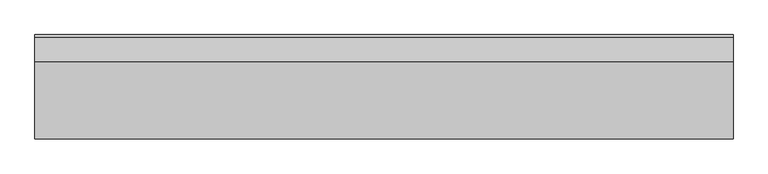
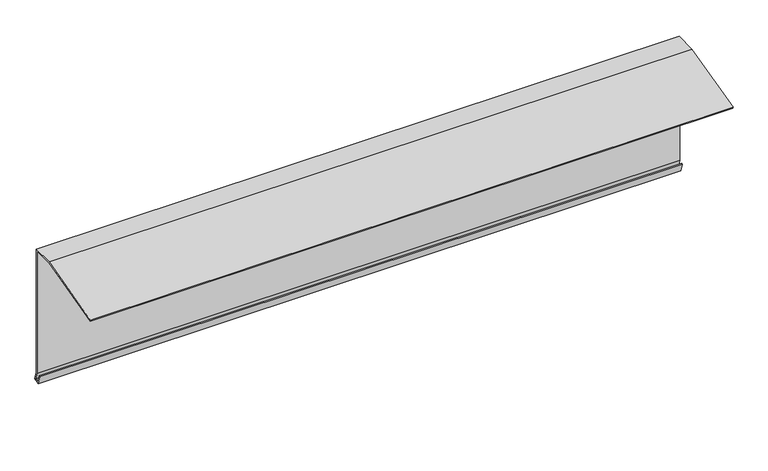
"""IFC4 building model written with IfcOpenShell, lengths in millimetres: proxy geometry, Flashing15:Flashing030:298298 : Flashing15:Flashing030:298298."""

from ifc_helpers import new_model, si_unit, frame, origin, place, context, project, spatial, polyline, outline, extrude, source, transform, mapped, element, save


def generic_models_658f80d1(model_context):
    return source(origin(), model_context, "Body", "SweptSolid", [
        extrude(outline(polyline([(2291.0928603, 44681.4656787), (2513.0807173, 44738.1803898), (2581.9034767, 44738.1803898), (2581.9034767, 44333.7602228), (2590.1892257, 44306.7687568), (2572.6272365, 44301.3776367), (2564.1057522, 44328.9010742), (2567.9268046, 44330.0841037), (2575.2697064, 44306.3673555), (2585.1972442, 44309.4000801), (2577.9034767, 44333.1600896), (2577.9034767, 44734.1803898), (2513.5836118, 44734.1803898), (2292.082999, 44677.5901625), (2291.0928603, 44681.4656787)])), frame((11247.1557516, 0.0, 0.0), z_axis=(1.0, 0.0, 0.0), x_axis=(0.0, 1.0, 0.0)), (0.0, 0.0, 1.0), 1999.85),
    ])


if __name__ == "__main__":
    model = new_model("IFC4")
    model_context = context("Model", 3, world=origin())
    ifc_project = project(units=[si_unit("LENGTHUNIT", "METRE", prefix="MILLI")], contexts=[model_context])
    site = spatial("IfcSite", under=ifc_project)
    building = spatial("IfcBuilding", under=site)
    placement = place(None, origin())
    generic_models_shape = generic_models_658f80d1(model_context)
    element("IfcBuildingElementProxy", 1, Name="Flashing15:Flashing030:298298 : Flashing15:Flashing030:298298", ObjectType="Flashing15:Flashing030:298298 : Flashing15:Flashing030:298298", at=placement, inside=building, context=model_context, shape_type="MappedRepresentation", body=[
        mapped(generic_models_shape, transform((0.0, 0.0, 0.0), x_axis=(1.0, 0.0, 0.0), y_axis=(0.0, 1.0, 0.0), z_axis=(0.0, 0.0, 1.0))),
    ])
    save(model, "model.ifc")

# Revit data of these elements
# Type "Flashing15:Flashing030:298298 : Flashing15:Flashing030:298298"
#   NameOverride = "Flashing15:Flashing030:298298"
#   ObjectTypeOverride = "Flashing15:Flashing030"
#   Reference = "Flashing030"
#   Category = "Generic Models"
#   Tag = "298298"
# Element 1 (IfcBuildingElementProxy, "Flashing15:Flashing030:298298 : Flashing15:Flashing030:298298")
#   Materials on its faces: "BRAKE METAL EAVE TRIM TO MATCH STANDING SEAM COLOR"
# Materials
#   "BRAKE METAL EAVE TRIM TO MATCH STANDING SEAM COLOR": class "Unassigned", colour RGB 128 128 128, transparency 0, Cost = 0
